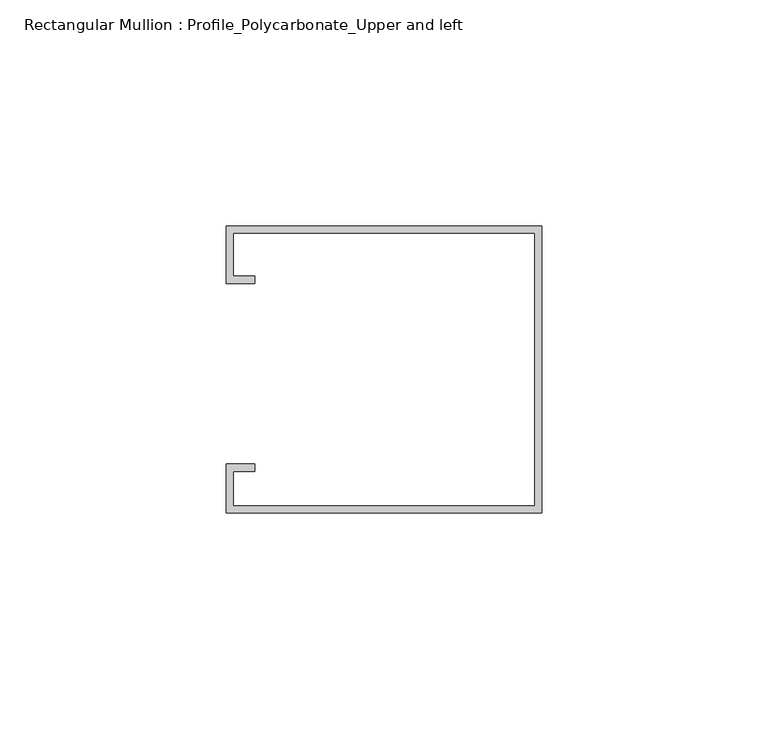
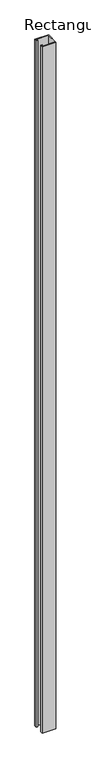
"""IFC4 building model written with IfcOpenShell, lengths in millimetres: member geometry, Rectangular Mullion : Profile_Polycarbonate_Upper and left."""

from ifc_helpers import new_model, si_unit, frame, origin, place, context, project, spatial, polyline, outline, extrude, source, transform, mapped, element, save


def rectangular_mullion_profile_polycarbonate_upper_and_left_b803591d(model_context):
    return source(origin(), model_context, "Body", "SweptSolid", [
        extrude(outline(polyline([(0.0, 32.7), (0.0, -30.8), (-69.85, -30.8), (-69.85, -20.0), (-63.5, -20.0), (-63.5, -21.5875), (-68.2625, -21.5875), (-68.2625, -29.2125), (-1.5875, -29.2125), (-1.5875, 31.1125), (-68.2625, 31.1125), (-68.2625, 21.5875), (-63.5, 21.5875), (-63.5, 20.0), (-69.85, 20.0), (-69.85, 32.7), (0.0, 32.7)])), frame((0.0, 0.0, -3695.7), z_axis=(0.0, 0.0, 1.0), x_axis=(1.0, 0.0, 0.0)), (0.0, 0.0, 1.0), 3695.7),
    ])


if __name__ == "__main__":
    model = new_model("IFC4")
    model_context = context("Model", 3, world=origin())
    ifc_project = project(units=[si_unit("LENGTHUNIT", "METRE", prefix="MILLI")], contexts=[model_context])
    site = spatial("IfcSite", under=ifc_project)
    building = spatial("IfcBuilding", under=site)
    placement = place(None, origin())
    rectangular_mullion_profile_polycarbonate_upper_and_left_shape = rectangular_mullion_profile_polycarbonate_upper_and_left_b803591d(model_context)
    element("IfcMember", 1, ObjectType="Rectangular Mullion : Profile_Polycarbonate_Upper and left", at=placement, inside=building, context=model_context, shape_type="MappedRepresentation", body=[
        mapped(rectangular_mullion_profile_polycarbonate_upper_and_left_shape, transform((0.0, 0.0, 0.0), x_axis=(1.0, 0.0, 0.0), y_axis=(0.0, 1.0, 0.0), z_axis=(0.0, 0.0, 1.0))),
    ])
    save(model, "model.ifc")

# Revit data of these elements
# Type "Rectangular Mullion : Profile_Polycarbonate_Upper and left"
#   built-in parameter 1007322 = 0.208333 (stored number, unit not read)
#   built-in parameter 1007321 = 0.00520833 (stored number, unit not read)
#   built-in parameter 1007320 = 0 (stored number, unit not read)
